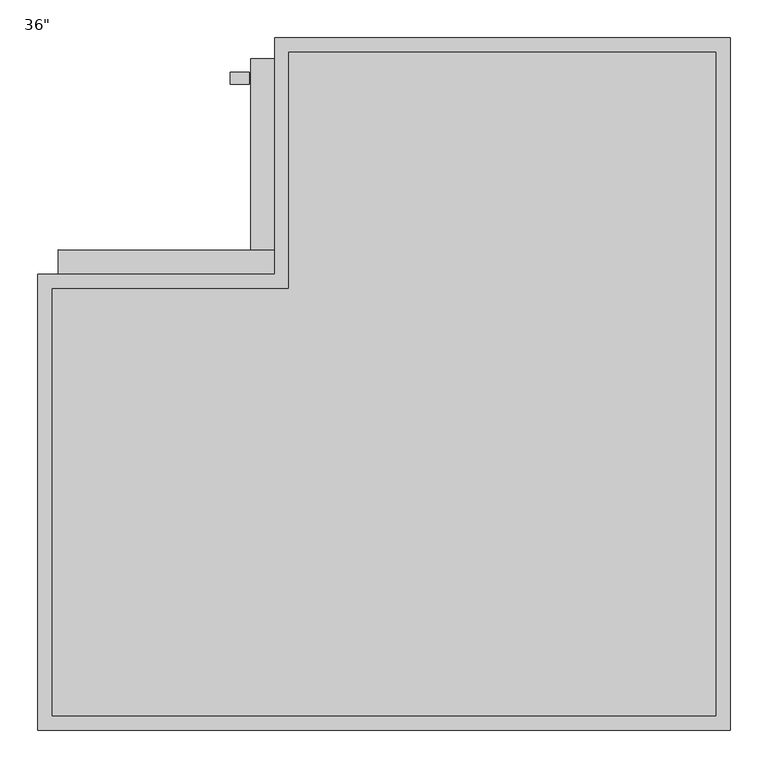
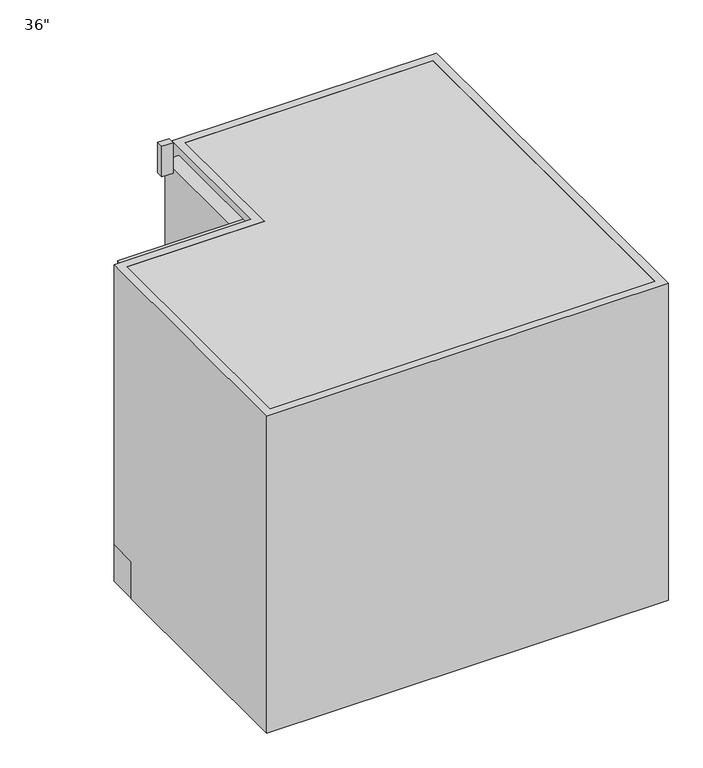
"""IFC4 building model written with IfcOpenShell, lengths in millimetres: furniture geometry."""

from ifc_helpers import new_model, si_unit, point, frame, frame_2d, origin, origin_with_axes, place, context, project, spatial, polyline, circle_curve, trimmed, segment, composite_curve, outline, extrude, faceted_brep, source, transform, mapped, element, save


def furniture_76622133(model_context):
    return source(origin(), model_context, "Body", "SolidModel", [
        extrude(outline(polyline([(-74.9665215, 633.9456685), (-75.0002151, 602.1956864), (-360.5187794, 602.4986834), (-360.4850858, 634.2486655), (-74.9665215, 633.9456685)])), frame((0.0, 0.0, 152.4), z_axis=(0.0, 0.0, 1.0), x_axis=(1.0, 0.0, 0.0)), (0.0, 0.0, 1.0), 590.55),
        faceted_brep([(526.7377049, 0.0, 762.0), (526.7377049, 914.4, 762.0), (-74.9833665, 914.4, 762.0), (-74.9833665, 602.3436184, 762.0), (-387.6622951, 602.3436184, 762.0), (-387.6622951, 0.0, 762.0), (507.6877049, 895.35, 762.0), (507.6877049, 19.05, 762.0), (-368.6122951, 19.05, 762.0), (-368.6122951, 583.2936184, 762.0), (-55.9333665, 583.2936184, 762.0), (-55.9333665, 895.35, 762.0), (-74.9833665, 914.4, 88.9), (-6.6622951, 914.4, 88.9), (-6.6622951, 895.35, 88.9), (-55.9333665, 895.35, 88.9), (-55.9333665, 583.2936184, 88.9), (-368.6122951, 583.2936184, 88.9), (-368.6122951, 534.0223805, 88.9), (-387.6622951, 534.0223805, 88.9), (-387.6622951, 602.3436184, 88.9), (-74.9833665, 602.3436184, 88.9), (-387.6622951, 0.0, 0.0), (526.7377049, 0.0, 0.0), (-387.6622951, 534.0223805, 0.0), (526.7377049, 914.4, 0.0), (-6.6622951, 914.4, 0.0), (507.6877049, 895.35, 88.9), (-368.6122951, 19.05, 88.9), (507.6877049, 19.05, 88.9), (-6.6622951, 534.0223805, 88.9), (-6.6622951, 534.0223805, 0.0)], [[[0, 1, 2, 3, 4, 5], [6, 7, 8, 9, 10, 11]], [[12, 13, 14, 15, 16, 17, 18, 19, 20, 21]], [[5, 22, 23, 0]], [[4, 20, 19, 24, 22, 5]], [[3, 21, 20, 4]], [[2, 12, 21, 3]], [[1, 25, 26, 13, 12, 2]], [[23, 25, 1, 0]], [[11, 15, 14, 27, 6]], [[10, 16, 15, 11]], [[9, 17, 16, 10]], [[8, 28, 18, 17, 9]], [[7, 29, 28, 8]], [[6, 27, 29, 7]], [[18, 28, 29, 27, 14, 30]], [[23, 22, 24, 31, 26, 25]], [[24, 19, 18, 30, 31]], [[31, 30, 14, 13, 26]]]),
        extrude(outline(polyline([(507.6877049, 19.05), (-368.6122951, 19.05), (-368.6122951, 602.3436184), (-74.9833665, 602.3436184), (-74.9833665, 895.35), (507.6877049, 895.35), (507.6877049, 19.05)])), frame((0.0, 0.0, 88.9), z_axis=(0.0, 0.0, 1.0), x_axis=(1.0, 0.0, 0.0)), (0.0, 0.0, 1.0), 19.05),
        extrude(outline(polyline([(526.7377049, 0.0), (-387.6622951, 0.0), (-387.6622951, 602.3436184), (-74.9833665, 602.3436184), (-74.9833665, 914.4), (526.7377049, 914.4), (526.7377049, 0.0)])), origin_with_axes(), (0.0, 0.0, 1.0), 762.0),
        extrude(outline(composite_curve([segment(trimmed(circle_curve(frame_2d((85.8132868, 441.5469651)), 19.05), [point((66.7632868, 441.5469651))], [point((104.8632868, 441.5469651))], False, "CARTESIAN"), True, "CONTINUOUS"), segment(trimmed(circle_curve(frame_2d((85.8132868, 441.5469651)), 19.05), [point((104.8632868, 441.5469651))], [point((66.7632868, 441.5469651))], False, "CARTESIAN"), True, "CONTINUOUS")], self_intersect=False)), origin_with_axes(), (0.0, 0.0, 1.0), 742.95),
        extrude(outline(composite_curve([segment(polyline([(-338.2830079, 566.4752307), (-36.9637809, 566.4752307), (-36.9637809, 867.1176746)]), True, "CONTINUOUS"), segment(trimmed(circle_curve(frame_2d((71.0113229, 457.5795168)), 423.5329098), [point((-36.9637809, 867.1176746))], [point((-338.2830079, 566.4752307))], False, "CARTESIAN"), True, "CONTINUOUS")], self_intersect=False)), frame((0.0, 0.0, 203.2), z_axis=(0.0, 0.0, 1.0), x_axis=(1.0, 0.0, 0.0)), (0.0, 0.0, 1.0), 45.0692226),
        extrude(outline(polyline([(-108.2622951, 853.255371), (-133.6622951, 853.255371), (-133.6622951, 869.0436184), (-108.2622951, 869.0436184), (-108.2622951, 853.255371)])), frame((0.0, 0.0, 732.086599), z_axis=(0.0, 0.0, 1.0), x_axis=(1.0, 0.0, 0.0)), (0.0, 0.0, 1.0), 73.5640045),
        extrude(outline(polyline([(-74.9833665, 886.7884981), (-74.9833665, 634.3478814), (-106.5244839, 634.3478814), (-106.5244839, 886.7884981), (-74.9833665, 886.7884981)])), frame((0.0, 0.0, 152.4), z_axis=(0.0, 0.0, 1.0), x_axis=(1.0, 0.0, 0.0)), (0.0, 0.0, 1.0), 590.55),
    ])


if __name__ == "__main__":
    model = new_model("IFC4")
    model_context = context("Model", 3, world=origin())
    ifc_project = project(units=[si_unit("LENGTHUNIT", "METRE", prefix="MILLI")], contexts=[model_context])
    site = spatial("IfcSite", under=ifc_project)
    building = spatial("IfcBuilding", under=site)
    placement = place(None, origin())
    furniture_shape = furniture_76622133(model_context)
    element("IfcFurniture", 1, ObjectType="36039039_Lazy_Susan_Base_Corner_Cabinet_with_ONE_rotating_shelf_14808 (1) : 36\"", at=placement, inside=building, context=model_context, shape_type="MappedRepresentation", body=[
        mapped(furniture_shape, transform((0.0, 0.0, 0.0), x_axis=(1.0, 0.0, 0.0), y_axis=(0.0, 1.0, 0.0), z_axis=(0.0, 0.0, 1.0))),
    ])
    save(model, "model.ifc")

# Revit data of these elements
# Type "36039039_Lazy_Susan_Base_Corner_Cabinet_with_ONE_rotating_shelf_14808 (1) : 36\""
#   Assembly Code = "C1030410"
#   Depth = 3' - 0"
#   Height = 2' - 6"
#   Toe Height = 0' - 3 1/2"
#   Width = 3' - 0"
#   Cabinet Material = Red Oak Low Gloss
#   Door/Drawer Material = none
#   Default Elevation = 0
# Element 1 (IfcFurniture, "36039039_Lazy_Susan_Base_Corner_Cabinet_with_ONE_rotating_shelf_14808 (1) : 36\"")
#   Materials on its faces: "Red Oak Low Gloss", "Cabinets", "Poche"
# Materials
#   "Red Oak Low Gloss": class "Generic", colour RGB 127 127 127, transparency 0, Cost = 0
#   "Cabinets": class "Miscellaneous", colour RGB 249 249 249, transparency 0
#   "Poche": class "System", colour RGB 0 0 255, transparency 0, Cost = 0
